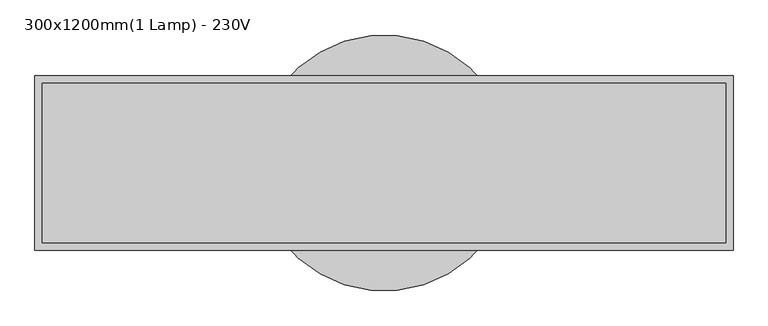
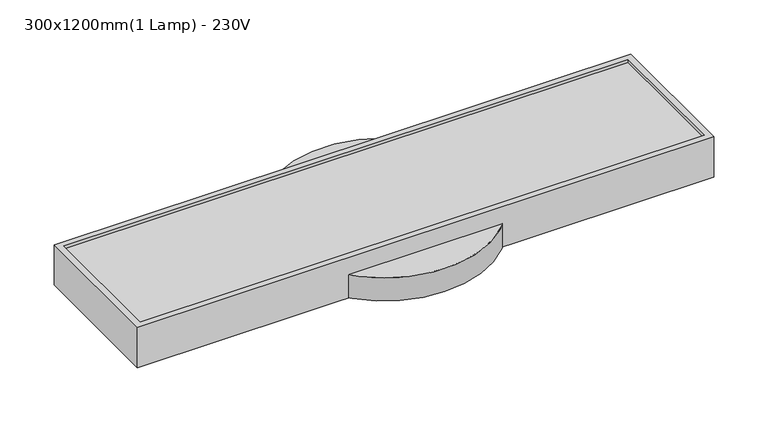
"""IFC4 building model written with IfcOpenShell, lengths in millimetres: light fixture geometry, Ceiling Light - Linear Box emergency light 300x1200mm 1Lamp 230 v : 300x1200mm(1 Lamp) - 230V."""

from ifc_helpers import new_model, si_unit, point, frame, frame_2d, origin, origin_with_axes, place, context, project, spatial, polyline, circle_curve, trimmed, segment, composite_curve, outline, extrude, source, transform, mapped, element, save


def light_fixture_300x1200mm_1_lamp_230v_5a723bfd(model_context):
    return source(origin(), model_context, "Body", "SweptSolid", [
        extrude(outline(composite_curve([segment(trimmed(circle_curve(frame_2d((0.0, -150.0)), 220.0), [point((-220.0, -150.0))], [point((220.0, -150.0))], False, "CARTESIAN"), True, "CONTINUOUS"), segment(trimmed(circle_curve(frame_2d((0.0, -150.0)), 220.0), [point((220.0, -150.0))], [point((-220.0, -150.0))], False, "CARTESIAN"), True, "CONTINUOUS")], self_intersect=False)), origin_with_axes(), (0.0, 0.0, 1.0), 50.8),
        extrude(outline(polyline([(587.3, -12.7), (587.3, -287.3), (-587.3, -287.3), (-587.3, -12.7), (587.3, -12.7)])), frame((0.0, 0.0, 76.2), z_axis=(0.0, 0.0, 1.0), x_axis=(1.0, 0.0, 0.0)), (0.0, 0.0, 1.0), 6.35),
        extrude(outline(polyline([(600.0, 0.0), (600.0, -300.0), (-600.0, -300.0), (-600.0, 0.0), (600.0, 0.0)]), holes=[polyline([(587.3, -12.7), (-587.3, -12.7), (-587.3, -287.3), (587.3, -287.3), (587.3, -12.7)])]), origin_with_axes(), (0.0, 0.0, 1.0), 88.9),
    ])


if __name__ == "__main__":
    model = new_model("IFC4")
    model_context = context("Model", 3, world=origin())
    ifc_project = project(units=[si_unit("LENGTHUNIT", "METRE", prefix="MILLI")], contexts=[model_context])
    site = spatial("IfcSite", under=ifc_project)
    building = spatial("IfcBuilding", under=site)
    placement = place(None, origin())
    light_fixture_300x1200mm_1_lamp_230v_shape = light_fixture_300x1200mm_1_lamp_230v_5a723bfd(model_context)
    element("IfcLightFixture", 1, ObjectType="Ceiling Light - Linear Box emergency light 300x1200mm 1Lamp 230 v : 300x1200mm(1 Lamp) - 230V", at=placement, inside=building, context=model_context, shape_type="MappedRepresentation", body=[
        mapped(light_fixture_300x1200mm_1_lamp_230v_shape, transform((0.0, 0.0, 0.0), x_axis=(1.0, 0.0, 0.0), y_axis=(0.0, 1.0, 0.0), z_axis=(0.0, 0.0, 1.0))),
    ])
    save(model, "model.ifc")

# Revit data of these elements
# Type "Ceiling Light - Linear Box emergency light 300x1200mm 1Lamp 230 v : 300x1200mm(1 Lamp) - 230V"
#   Type Mark = "Ceiling Light - Linear Box emergency light 300x1200mm 1Lamp 230 v"
#   Classification.OmniClass.21.Number = "21-04 50 40 50"
#   Classification.OmniClass.21.Description = "Lighting Fixtures"
#   Classification.UniFormat.II.Description = "Lighting Fixtures"
#   Classification.OmniClass.23.Number = "23-35 47 13"
#   Classification.OmniClass.23.Description = "Emergency Lighting"
#   Classification.UniFormat.II.Number = "D5040.50"
#   COBie.Type.CreatedBy = "info@mma.ie"
#   COBie.Type.CreatedOn = "2017-07-25T10:15:16"
#   COBie.Type.Name = "Ceiling Light - Linear Box emergency light 300x1200mm 1Lamp 230 v"
#   COBie.Type.Category = "23-35 47 13 : Emergency Lighting"
#   COBie.Type.Description = "Ceiling Light - Linear Box emergency light 300x1200mm 1Lamp 230 v_300x1200mm(1 Lamp) - 230V"
#   COBie.Type.AssetType = "Fixed"
#   COBie.Type.Manufacturer = ""
#   COBie.Type.ModelNumber = ""
#   Photometric Web File = "1x41T12.ies"
#   Lamp = "T-12"
#   Keynote = "26 52 00.A"
#   Assembly Code = "D5020210"
#   COBie.Type.ReplacementCost = 0
#   Width 1 = 150 mm
#   Wattage = 40 W
#   built-in parameter 1150110 = 1 (stored number, unit not read)
#   built-in parameter 1114217 = 0.88 (stored number, unit not read)
#   built-in parameter 1150109 = 1 (stored number, unit not read)
#   built-in parameter 1150113 = 1 (stored number, unit not read)
#   Tilt Angle = -90.00°
#   Lumens = 3150 lm
#   built-in parameter 1150115 = 1 (stored number, unit not read)
#   built-in parameter 1150105 = 250.669 (stored number, unit not read)
#   Length1 = 600 mm
#   built-in parameter 1150112 = 1 (stored number, unit not read)
#   built-in parameter 1150114 = 1 (stored number, unit not read)
#   built-in parameter 1150107 = 4230 (stored number, unit not read)
#   built-in parameter 1150106 = 2.50669 (stored number, unit not read)
#   Emit from Rectangle Width = 274 mm
#   Emit from Rectangle Length = 1174 mm
#   built-in parameter 1150104 = 7.31611 (stored number, unit not read)
#   Default Elevation = 1200 mm
#   C.L.E - Width = 300 mm
#   C.L.E - Length = 1200 mm
#   C.L.E - Depth = 88.9 mm
#   Box Width = 300 mm
#   Box Length = 1200 mm
#   Ballast Voltage = 230 V
#   built-in parameter 1114218 = 0.88 (stored number, unit not read)
#   built-in parameter 1150133 = 10 (stored number, unit not read)
#   Apparent Load = 40 VA
#   COBie.Type = yes
#   built-in parameter 1150134 = 8
#   built-in parameter 1150137 = 1
#   Color Filter = 16777215
#   built-in parameter 1140040 [instance default] = 1
#   Ballast Number of Poles = 1
#   black = Phase - Demo
#   Load Classification = Lighting - Dwelling Unit
#   Light Box Material = Metal - Paint Finish - Ivory, Glossy
#   Diffuser Material = Glass - White, High Luminance
#   Emit Shape Visible in Rendering = no
#   Dimming Lamp Color Temperature Shift = (empty or 0)
# Element 1 (IfcLightFixture, "Ceiling Light - Linear Box emergency light 300x1200mm 1Lamp 230 v : 300x1200mm(1 Lamp) - 230V")
#   Materials on its faces: "Phase - Demo", "Glass - White, High Luminance"
# Materials
#   "Phase - Demo": class "System", colour RGB 255 0 0, transparency 0.4
#   "Metal - Paint Finish - Ivory, Glossy": class "Paint", colour RGB 247 247 239, transparency 0, Comments = "Rendering appearance not upgraded "
#   "Glass - White, High Luminance": class "Glass", colour RGB 249 250 249, transparency 0.8
